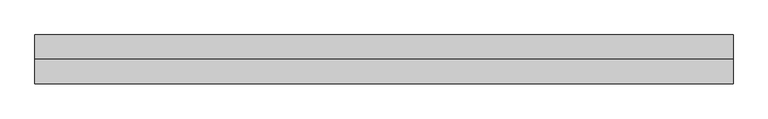
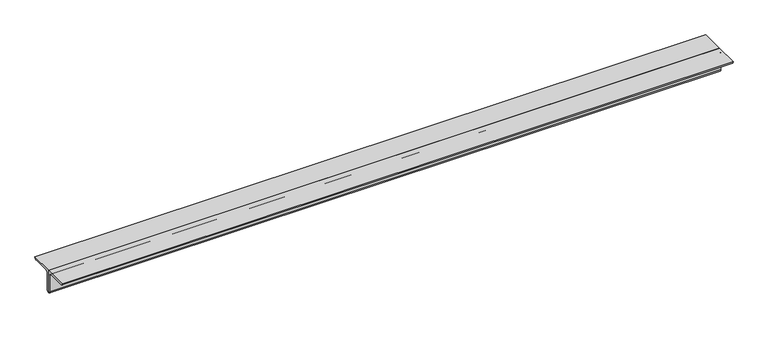
"""IFC4 building model written with IfcOpenShell, lengths in millimetres: member geometry, 0123_Steel Framing_2Ls-KSD3502 : H_SB_AR_S03_2Ls-130x130x12_HBR1."""

import ifcopenshell
import ifcopenshell.guid

model = None  # the IFC model being written
_history = None  # IfcOwnerHistory: only IFC2X3 demands one
_inside = {}  # id of a spatial element -> (the spatial element, [elements in it])
_under = {}  # id of a project, library or spatial element -> (it, [spatial elements below it])
_declared = {}  # id of a project -> (the project, [libraries it declares])
_typed = {}  # id of a type object -> (the type object, [elements of that type])
_made_of = {}  # id of a material, layer set ... -> (it, [elements and type objects made of it])


def new_model(schema):
    """Start an empty IFC model of exactly this schema.

    Asked for "IFC4X3", IfcOpenShell would pick the latest addendum, in which some entities
    have other attributes; the version numbers below select the first issue.
    IFC2X3 requires an IfcOwnerHistory on every rooted entity: one is made here for all.
    """
    global model, _history
    if schema == "IFC4X3":
        model = ifcopenshell.file(schema_version=(4, 3, 0, 0))
    else:
        model = ifcopenshell.file(schema=schema)
    _inside.clear()
    _under.clear()
    _declared.clear()
    _typed.clear()
    _made_of.clear()
    _history = None
    if model.schema == "IFC2X3":
        org = make("IfcOrganization", Name="unknown")
        user = make(
            "IfcPersonAndOrganization",
            ThePerson=make("IfcPerson", FamilyName="unknown"),
            TheOrganization=org,
        )
        app = make(
            "IfcApplication",
            ApplicationDeveloper=org,
            Version="unknown",
            ApplicationFullName="unknown",
            ApplicationIdentifier="unknown",
        )
        _history = make(
            "IfcOwnerHistory",
            OwningUser=user,
            OwningApplication=app,
            ChangeAction="ADDED",
            CreationDate=0,
        )
    return model


def make(cls, **values):
    """One entity of the class cls with the attributes given. An attribute that is None is left unset."""
    return model.create_entity(
        cls, **{name: value for name, value in values.items() if value is not None}
    )


def rooted(cls, **values):
    """An entity with a GlobalId (a new one), such as an element, a storey or a relation."""
    return make(cls, GlobalId=ifcopenshell.guid.new(), OwnerHistory=_history, **values)


def si_unit(unit_type, name, prefix=None):
    """IfcSIUnit, for example si_unit("LENGTHUNIT", "METRE", prefix="MILLI")."""
    return make("IfcSIUnit", UnitType=unit_type, Prefix=prefix, Name=name)


def assignment(units):
    """IfcUnitAssignment: the units of a project."""
    return None if units is None else make("IfcUnitAssignment", Units=units)


def point(xyz):
    """IfcCartesianPoint."""
    return None if xyz is None else make("IfcCartesianPoint", Coordinates=xyz)


def direction(xyz):
    """IfcDirection."""
    return None if xyz is None else make("IfcDirection", DirectionRatios=xyz)


def frame(location, z_axis=None, x_axis=None):
    """IfcAxis2Placement3D, a coordinate frame: its origin and axes. An axis left out is left unset."""
    return make(
        "IfcAxis2Placement3D",
        Location=point(location),
        Axis=direction(z_axis),
        RefDirection=direction(x_axis),
    )


def frame_2d(location, x_axis=None):
    """IfcAxis2Placement2D, a coordinate frame in the plane: its origin and x axis."""
    return make(
        "IfcAxis2Placement2D", Location=point(location), RefDirection=direction(x_axis)
    )


def origin():
    """The frame at (0, 0, 0) with its axes left unset."""
    return frame((0.0, 0.0, 0.0))


def place(relative_to, where):
    """IfcLocalPlacement: puts the frame where relative to a parent placement (None: the world)."""
    return make(
        "IfcLocalPlacement", PlacementRelTo=relative_to, RelativePlacement=where
    )


def context(
    kind, dimensions, precision=None, world=None, true_north=None, identifier=None
):
    """IfcGeometricRepresentationContext, for example the 3D "Model" context."""
    return make(
        "IfcGeometricRepresentationContext",
        ContextIdentifier=identifier,
        ContextType=kind,
        CoordinateSpaceDimension=dimensions,
        Precision=precision,
        WorldCoordinateSystem=world,
        TrueNorth=true_north,
    )


def project(units=None, contexts=None):
    """IfcProject with its units and contexts."""
    return rooted(
        "IfcProject",
        Name="project",
        RepresentationContexts=contexts,
        UnitsInContext=assignment(units),
    )


def spatial(cls, under=None, at=None, **own):
    """A site, building, storey or space (cls), placed at a placement, below another one or the project."""
    s = rooted(cls, ObjectPlacement=at, **own)
    if under is not None:
        _under.setdefault(under.id(), (under, []))[1].append(s)
    return s


def polyline(points):
    """IfcPolyline through the points."""
    return make("IfcPolyline", Points=[point(p) for p in points])


def circle_curve(where, radius):
    """IfcCircle in the frame where."""
    return make("IfcCircle", Position=where, Radius=radius)


def trimmed(basis, trim1, trim2, sense, master):
    """IfcTrimmedCurve: the piece of a basis curve between two trims."""
    return make(
        "IfcTrimmedCurve",
        BasisCurve=basis,
        Trim1=trim1,
        Trim2=trim2,
        SenseAgreement=sense,
        MasterRepresentation=master,
    )


def segment(curve, same_sense, transition):
    """IfcCompositeCurveSegment."""
    return make(
        "IfcCompositeCurveSegment",
        Transition=transition,
        SameSense=same_sense,
        ParentCurve=curve,
    )


def composite_curve(segments, self_intersect=None):
    """IfcCompositeCurve: segments joined end to end."""
    return make("IfcCompositeCurve", Segments=segments, SelfIntersect=self_intersect)


def outline(outer, holes=None, kind="AREA"):
    """IfcArbitraryClosedProfileDef: a profile drawn as a closed curve; with holes, ...WithVoids."""
    if holes is None:
        return make("IfcArbitraryClosedProfileDef", ProfileType=kind, OuterCurve=outer)
    return make(
        "IfcArbitraryProfileDefWithVoids",
        ProfileType=kind,
        OuterCurve=outer,
        InnerCurves=holes,
    )


def extrude(swept, where, along, depth):
    """IfcExtrudedAreaSolid: the profile swept, set in the frame where, extruded along a direction by depth."""
    return make(
        "IfcExtrudedAreaSolid",
        SweptArea=swept,
        Position=where,
        ExtrudedDirection=direction(along),
        Depth=depth,
    )


def shape(context_of_items, identifier, shape_type, items):
    """IfcShapeRepresentation: the items that make up one representation, for example the "Body"."""
    return make(
        "IfcShapeRepresentation",
        ContextOfItems=context_of_items,
        RepresentationIdentifier=identifier,
        RepresentationType=shape_type,
        Items=items,
    )


def source(mapping_origin, context_of_items, identifier, shape_type, items):
    """IfcRepresentationMap: a shape defined once, which mapped items show again and again."""
    return make(
        "IfcRepresentationMap",
        MappingOrigin=mapping_origin,
        MappedRepresentation=shape(context_of_items, identifier, shape_type, items),
    )


def transform(
    local_origin,
    x_axis=None,
    y_axis=None,
    z_axis=None,
    scale=None,
    scale2=None,
    scale3=None,
    uniform=True,
):
    """IfcCartesianTransformationOperator3D, or its non-uniform kind. x_axis, y_axis, z_axis: its Axis1, 2, 3."""
    if uniform:
        return make(
            "IfcCartesianTransformationOperator3D",
            Axis1=direction(x_axis),
            Axis2=direction(y_axis),
            LocalOrigin=point(local_origin),
            Scale=scale,
            Axis3=direction(z_axis),
        )
    return make(
        "IfcCartesianTransformationOperator3DnonUniform",
        Axis1=direction(x_axis),
        Axis2=direction(y_axis),
        LocalOrigin=point(local_origin),
        Scale=scale,
        Axis3=direction(z_axis),
        Scale2=scale2,
        Scale3=scale3,
    )


def mapped(mapping_source, mapping_target):
    """IfcMappedItem: shows the shape of a source again, moved by a transform."""
    return make(
        "IfcMappedItem", MappingSource=mapping_source, MappingTarget=mapping_target
    )


def made_of(thing, what):
    """Note that an element or type object is made of a material, layer set ...; save() writes the relation."""
    if what is not None:
        _made_of.setdefault(what.id(), (what, []))[1].append(thing)
    return thing


def element(
    cls,
    number,
    at=None,
    inside=None,
    cuts=None,
    type_object=None,
    material=None,
    context=None,
    identifier="Body",
    shape_type=None,
    held_by="IfcProductDefinitionShape",
    body=None,
    shapes=None,
    **own,
):
    """One element of the class cls, such as IfcWall. Its Tag is "e" and its number.

    at: its placement. inside: the storey or other place that contains it. cuts: it is an
    opening in that element (IfcRelVoidsElement). A single representation is given by context,
    identifier, shape_type and body (its items); several are given by shapes. held_by: the class
    of the entity that holds the representations. save() writes the other relations.
    """
    e = rooted(cls, Tag="e%d" % number, ObjectPlacement=at, **own)
    if body is not None:
        shapes = [shape(context, identifier, shape_type, body)]
    if shapes is not None:
        e.Representation = make(held_by, Representations=shapes)
    if inside is not None:
        _inside.setdefault(inside.id(), (inside, []))[1].append(e)
    if cuts is not None:
        rooted(
            "IfcRelVoidsElement", RelatingBuildingElement=cuts, RelatedOpeningElement=e
        )
    if type_object is not None:
        _typed.setdefault(type_object.id(), (type_object, []))[1].append(e)
    return made_of(e, material)


def aggregate(whole, parts):
    """IfcRelAggregates: a whole, such as a stair, and the parts it consists of."""
    return rooted("IfcRelAggregates", RelatingObject=whole, RelatedObjects=parts)


def save(model, path):
    """Write the relations noted so far, then the file.

    IfcRelAggregates (storeys below a building ...), IfcRelContainedInSpatialStructure (elements
    in a storey), IfcRelDefinesByType, IfcRelAssociatesMaterial and IfcRelDeclares: one each for
    every whole, place, type object, material and project.
    """
    for whole, parts in _under.values():
        aggregate(whole, parts)
    for where, things in _inside.values():
        rooted(
            "IfcRelContainedInSpatialStructure",
            RelatedElements=things,
            RelatingStructure=where,
        )
    for kind, things in _typed.values():
        rooted("IfcRelDefinesByType", RelatedObjects=things, RelatingType=kind)
    for what, things in _made_of.values():
        rooted("IfcRelAssociatesMaterial", RelatedObjects=things, RelatingMaterial=what)
    for by, libraries in _declared.values():
        rooted("IfcRelDeclares", RelatingContext=by, RelatedDefinitions=libraries)
    model.write(path)


def member_70dd3ef8(model_context):
    return source(origin(), model_context, "Body", "SweptSolid", [
        extrude(outline(composite_curve([segment(polyline([(0.0, 36.4), (0.0, -93.6)]), True, "CONTINUOUS"), segment(trimmed(circle_curve(frame_2d((0.0, -81.6)), 12.0), [point((0.0, -93.6))], [point((-12.0, -81.6))], False, "CARTESIAN"), True, "CONTINUOUS"), segment(polyline([(-12.0, -81.6), (-12.0, 12.4)]), True, "CONTINUOUS"), segment(trimmed(circle_curve(frame_2d((-24.0, 12.4)), 12.0), [point((-12.0, 12.4))], [point((-24.0, 24.4))], True, "CARTESIAN"), True, "CONTINUOUS"), segment(polyline([(-24.0, 24.4), (-118.0, 24.4)]), True, "CONTINUOUS"), segment(trimmed(circle_curve(frame_2d((-118.0, 36.4)), 12.0), [point((-118.0, 24.4))], [point((-130.0, 36.4))], False, "CARTESIAN"), True, "CONTINUOUS"), segment(polyline([(-130.0, 36.4), (0.0, 36.4)]), True, "CONTINUOUS")], self_intersect=False)), frame((-1844.6975967, 0.0, 0.0), z_axis=(1.0, 0.0, 0.0), x_axis=(0.0, 1.0, 0.0)), (0.0, 0.0, 1.0), 3701.6272171),
        extrude(outline(composite_curve([segment(polyline([(0.0, 36.4), (130.0, 36.4)]), True, "CONTINUOUS"), segment(trimmed(circle_curve(frame_2d((118.0, 36.4)), 12.0), [point((130.0, 36.4))], [point((118.0, 24.4))], False, "CARTESIAN"), True, "CONTINUOUS"), segment(polyline([(118.0, 24.4), (24.0, 24.4)]), True, "CONTINUOUS"), segment(trimmed(circle_curve(frame_2d((24.0, 12.4)), 12.0), [point((24.0, 24.4))], [point((12.0, 12.4))], True, "CARTESIAN"), True, "CONTINUOUS"), segment(polyline([(12.0, 12.4), (12.0, -81.6)]), True, "CONTINUOUS"), segment(trimmed(circle_curve(frame_2d((0.0, -81.6)), 12.0), [point((12.0, -81.6))], [point((0.0, -93.6))], False, "CARTESIAN"), True, "CONTINUOUS"), segment(polyline([(0.0, -93.6), (0.0, 36.4)]), True, "CONTINUOUS")], self_intersect=False)), frame((-1844.6975967, 0.0, 0.0), z_axis=(1.0, 0.0, 0.0), x_axis=(0.0, 1.0, 0.0)), (0.0, 0.0, 1.0), 3701.6272171),
    ])


if __name__ == "__main__":
    model = new_model("IFC4")
    model_context = context("Model", 3, world=origin())
    ifc_project = project(units=[si_unit("LENGTHUNIT", "METRE", prefix="MILLI")], contexts=[model_context])
    site = spatial("IfcSite", under=ifc_project)
    building = spatial("IfcBuilding", under=site)
    placement = place(None, origin())
    member_shape = member_70dd3ef8(model_context)
    element("IfcMember", 1, ObjectType="0123_Steel Framing_2Ls-KSD3502 : H_SB_AR_S03_2Ls-130x130x12_HBR1", at=placement, inside=building, context=model_context, shape_type="MappedRepresentation", body=[
        mapped(member_shape, transform((0.0, 0.0, 0.0), x_axis=(1.0, 0.0, 0.0), y_axis=(0.0, 1.0, 0.0), z_axis=(0.0, 0.0, 1.0))),
    ])
    save(model, "model.ifc")

# Revit data of these elements
# Type "0123_Steel Framing_2Ls-KSD3502 : H_SB_AR_S03_2Ls-130x130x12_HBR1"
#   Assembly Code = "B10"
#   Legs = "SLBB"
#   W = 8.97
#   Perimeter = 1.04 m²/m
#   Nominal Weight = 46.80 kgf/m
#   Length [instance default] = 1000 mm
#   Space = 0 mm
#   b = 130 mm
#   d = 130 mm
#   t = 12 mm
#   y = 36.4 mm
#   A = 0.005952 m²
#   Structural Material [instance default] = Steel ASTM A36
# Element 1 (IfcMember, "0123_Steel Framing_2Ls-KSD3502 : H_SB_AR_S03_2Ls-130x130x12_HBR1")
#   Structural Material = Steel, 45-345
#   Materials on its faces: "Steel, 45-345"
# Materials
#   "Steel ASTM A36": class "Metal", colour RGB 199 199 199, transparency 0, Description = "Structural steel, ASTM A36 Grade B, mill finish", Cost = 0
#   "Steel, 45-345": class "Metal", colour RGB 189 187 185, transparency 0, Description = "Steel 345 MPa", Cost = 0
